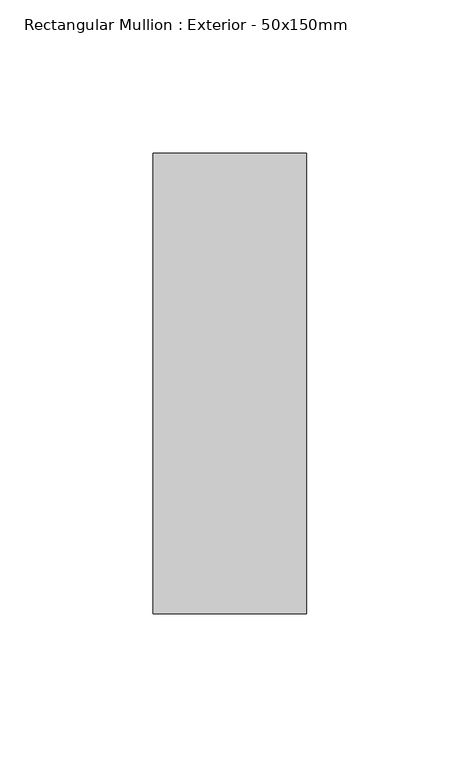
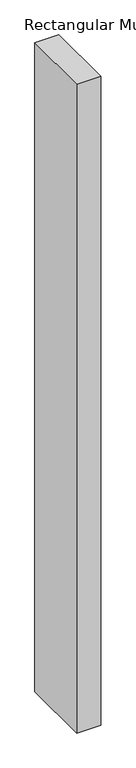
"""IFC4 building model written with IfcOpenShell, lengths in millimetres: member geometry, Rectangular Mullion : Exterior - 50x150mm."""

from ifc_helpers import new_model, si_unit, frame, origin, place, context, project, spatial, polyline, outline, extrude, source, transform, mapped, element, save


def rectangular_mullion_exterior_50x150mm_b89aef2e(model_context):
    return source(origin(), model_context, "Body", "SweptSolid", [
        extrude(outline(polyline([(0.0, 0.0), (0.0, -150.0), (-50.0, -150.0), (-50.0, 0.0), (0.0, 0.0)])), frame((0.0, 0.0, -1425.0000002), z_axis=(0.0, 0.0, 1.0), x_axis=(1.0, 0.0, 0.0)), (0.0, 0.0, 1.0), 1425.0000002),
    ])


if __name__ == "__main__":
    model = new_model("IFC4")
    model_context = context("Model", 3, world=origin())
    ifc_project = project(units=[si_unit("LENGTHUNIT", "METRE", prefix="MILLI")], contexts=[model_context])
    site = spatial("IfcSite", under=ifc_project)
    building = spatial("IfcBuilding", under=site)
    placement = place(None, origin())
    rectangular_mullion_exterior_50x150mm_shape = rectangular_mullion_exterior_50x150mm_b89aef2e(model_context)
    element("IfcMember", 1, ObjectType="Rectangular Mullion : Exterior - 50x150mm", at=placement, inside=building, context=model_context, shape_type="MappedRepresentation", body=[
        mapped(rectangular_mullion_exterior_50x150mm_shape, transform((0.0, 0.0, 0.0), x_axis=(1.0, 0.0, 0.0), y_axis=(0.0, 1.0, 0.0), z_axis=(0.0, 0.0, 1.0))),
    ])
    save(model, "model.ifc")

# Revit data of these elements
# Type "Rectangular Mullion : Exterior - 50x150mm"
#   built-in parameter 1007351 = -0.246063 (stored number, unit not read)
#   built-in parameter 1007304 = 0.492126 (stored number, unit not read)
#   built-in parameter 1007301 = 0.082021 (stored number, unit not read)
#   built-in parameter 1007300 = 0.082021 (stored number, unit not read)
# Element 1 (IfcMember, "Rectangular Mullion : Exterior - 50x150mm")
#   Materials on its faces: "Default Frame/Mullion (Interior/Exterior)"
# Materials
#   "Default Frame/Mullion (Interior/Exterior)": class "Generic", colour RGB 205 205 205, transparency 0, Description = "Udefineret karm/ramme materiale", Cost = 0
